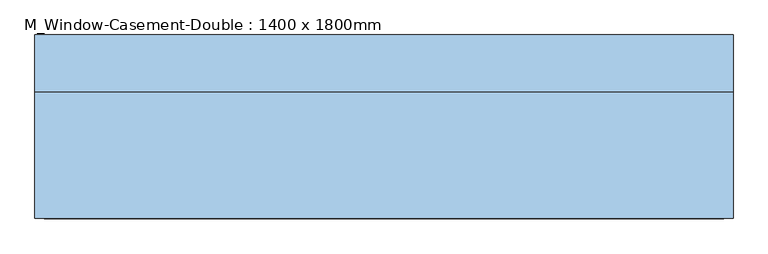
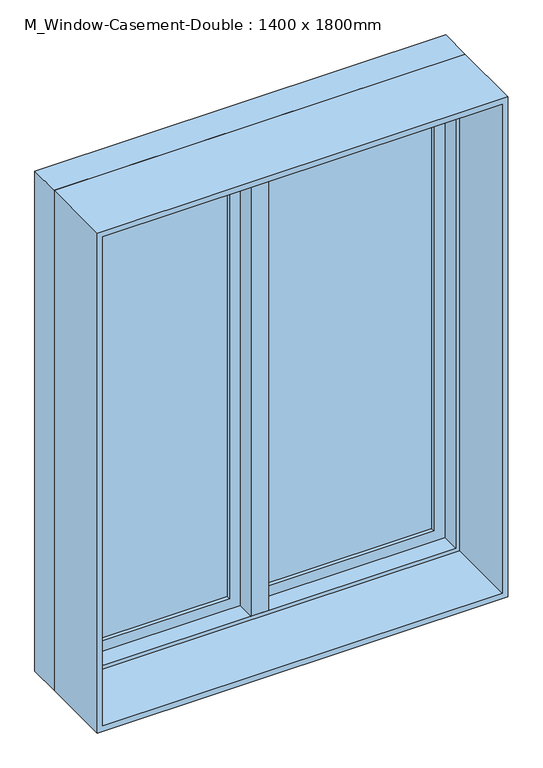
"""IFC4 building model written with IfcOpenShell, lengths in millimetres: window geometry, M_Window-Casement-Double : 1400 x 1800mm."""

from ifc_helpers import new_model, si_unit, frame, origin, place, context, project, spatial, polyline, outline, extrude, faceted_brep, source, transform, mapped, element, save


def m_window_casement_double_1400_x_1800mm_1c3ec30c(model_context):
    return source(origin(), model_context, "Body", "SolidModel", [
        faceted_brep([(668.25, 142.75, 2668.25), (668.25, 79.25, 2668.25), (-668.25, 79.25, 2668.25), (-668.25, 142.75, 2668.25), (687.3, 193.55, 2687.3), (687.3, 142.75, 2687.3), (-687.3, 142.75, 2687.3), (-687.3, 193.55, 2687.3), (700.0, 79.25, 2700.0), (700.0, 193.55, 2700.0), (-700.0, 193.55, 2700.0), (-700.0, 79.25, 2700.0), (-668.25, 79.25, 931.75), (-668.25, 142.75, 931.75), (-687.3, 142.75, 912.7), (-687.3, 193.55, 912.7), (-700.0, 193.55, 900.0), (-700.0, 79.25, 900.0), (668.25, 79.25, 931.75), (668.25, 142.75, 931.75), (687.3, 142.75, 912.7), (687.3, 193.55, 912.7), (700.0, 193.55, 900.0), (700.0, 79.25, 900.0)], [[[0, 1, 2, 3]], [[4, 5, 6, 7]], [[8, 9, 10, 11]], [[3, 2, 12, 13]], [[7, 6, 14, 15]], [[11, 10, 16, 17]], [[13, 12, 18, 19]], [[15, 14, 20, 21]], [[17, 16, 22, 23]], [[11, 17, 23, 8], [1, 18, 12, 2]], [[19, 18, 1, 0]], [[5, 20, 14, 6], [3, 13, 19, 0]], [[21, 20, 5, 4]], [[23, 22, 9, 8]], [[9, 22, 16, 10], [7, 15, 21, 4]]]),
        extrude(outline(polyline([(2700.0, -700.0), (900.0, -700.0), (900.0, 700.0), (2700.0, 700.0), (2700.0, -700.0)]), holes=[polyline([(2680.95, 680.95), (919.05, 680.95), (919.05, -680.95), (2680.95, -680.95), (2680.95, 680.95)])]), frame((0.0, -174.5, 0.0), z_axis=(0.0, 1.0, 0.0), x_axis=(0.0, 0.0, 1.0)), (0.0, 0.0, 1.0), 253.75),
        extrude(outline(polyline([(912.7, 687.3), (2687.3, 687.3), (2687.3, 9.525), (912.7, 9.525), (912.7, 687.3)]), holes=[polyline([(969.85, 66.675), (2630.15, 66.675), (2630.15, 630.15), (969.85, 630.15), (969.85, 66.675)])]), frame((0.0, 142.75, 0.0), z_axis=(0.0, 1.0, 0.0), x_axis=(0.0, 0.0, 1.0)), (0.0, 0.0, 1.0), 44.45),
        extrude(outline(polyline([(2687.3, -687.3), (912.7, -687.3), (912.7, -9.525), (2687.3, -9.525), (2687.3, -687.3)]), holes=[polyline([(2630.15, -66.675), (969.85, -66.675), (969.85, -630.15), (2630.15, -630.15), (2630.15, -66.675)])]), frame((0.0, 142.75, 0.0), z_axis=(0.0, 1.0, 0.0), x_axis=(0.0, 0.0, 1.0)), (0.0, 0.0, 1.0), 44.45),
        extrude(outline(polyline([(630.15, 174.5), (630.15, 168.15), (66.675, 168.15), (66.675, 174.5), (630.15, 174.5)])), frame((0.0, 0.0, 969.85), z_axis=(0.0, 0.0, 1.0), x_axis=(1.0, 0.0, 0.0)), (0.0, 0.0, 1.0), 1660.3),
        extrude(outline(polyline([(66.675, 155.45), (66.675, 161.8), (630.15, 161.8), (630.15, 155.45), (66.675, 155.45)])), frame((0.0, 0.0, 969.85), z_axis=(0.0, 0.0, 1.0), x_axis=(1.0, 0.0, 0.0)), (0.0, 0.0, 1.0), 1660.3),
        extrude(outline(polyline([(-66.675, 174.5), (-66.675, 168.15), (-630.15, 168.15), (-630.15, 174.5), (-66.675, 174.5)])), frame((0.0, 0.0, 969.85), z_axis=(0.0, 0.0, 1.0), x_axis=(1.0, 0.0, 0.0)), (0.0, 0.0, 1.0), 1660.3),
        extrude(outline(polyline([(-630.15, 155.45), (-630.15, 161.8), (-66.675, 161.8), (-66.675, 155.45), (-630.15, 155.45)])), frame((0.0, 0.0, 969.85), z_axis=(0.0, 0.0, 1.0), x_axis=(1.0, 0.0, 0.0)), (0.0, 0.0, 1.0), 1660.3),
        faceted_brep([(9.525, 193.55, 2687.3), (-9.525, 193.55, 2687.3), (-9.525, 142.75, 2687.3), (9.525, 142.75, 2687.3), (9.525, 193.55, 912.7), (9.525, 142.75, 912.7), (-9.525, 142.75, 912.7), (-9.525, 193.55, 912.7), (-9.525, 142.75, 931.75), (-9.525, 142.75, 2668.25), (-30.1625, 142.75, 931.75), (-30.1625, 142.75, 2668.25), (-30.1625, 79.25, 931.75), (-30.1625, 79.25, 2668.25), (30.1625, 79.25, 931.75), (30.1625, 79.25, 2668.25), (30.1625, 142.75, 931.75), (30.1625, 142.75, 2668.25), (9.525, 142.75, 931.75), (9.525, 142.75, 2668.25)], [[[0, 1, 2, 3]], [[4, 5, 6, 7]], [[1, 0, 4, 7]], [[2, 1, 7, 6, 8, 9]], [[9, 8, 10, 11]], [[11, 10, 12, 13]], [[13, 12, 14, 15]], [[15, 14, 16, 17]], [[17, 16, 18, 19]], [[0, 3, 19, 18, 5, 4]], [[18, 8, 6, 5]], [[9, 19, 3, 2]], [[8, 18, 16, 14, 12, 10]], [[19, 9, 11, 13, 15, 17]]]),
    ])


if __name__ == "__main__":
    model = new_model("IFC4")
    model_context = context("Model", 3, world=origin())
    ifc_project = project(units=[si_unit("LENGTHUNIT", "METRE", prefix="MILLI")], contexts=[model_context])
    site = spatial("IfcSite", under=ifc_project)
    building = spatial("IfcBuilding", under=site)
    placement = place(None, origin())
    m_window_casement_double_1400_x_1800mm_shape = m_window_casement_double_1400_x_1800mm_1c3ec30c(model_context)
    element("IfcWindow", 1, ObjectType="M_Window-Casement-Double : 1400 x 1800mm", at=placement, inside=building, context=model_context, shape_type="MappedRepresentation", body=[
        mapped(m_window_casement_double_1400_x_1800mm_shape, transform((0.0, 0.0, 0.0), x_axis=(1.0, 0.0, 0.0), y_axis=(0.0, 1.0, 0.0), z_axis=(0.0, 0.0, 1.0))),
    ])
    save(model, "model.ifc")

# Revit data of these elements
# Type "M_Window-Casement-Double : 1400 x 1800mm"
#   Type Mark = "27"
#   Fire Rating = "0.5h"
#   Assembly Code = "B2020100"
#   Analytic Construction = "Double glazing - domestic"
#   Frame Extension [instance default] = 6.35 mm
#   Window Inset [instance default] = 0 mm
#   Wall Thickness [instance default] = 150 mm
#   Interior Wall Closure [instance default] = 54.75 mm
#   Half Width = 700 mm
#   Visual Light Transmittance = 0.81
#   Thermal Resistance (R) = 0.319569 (m²·K)/W
#   Solar Heat Gain Coefficient = 0.76
#   Rough Width = 1415 mm
#   Rough Height = 1815 mm
#   Height = 1800 mm
#   Heat Transfer Coefficient (U) = 3.12929 W/(m²·K)
#   Exterior Wall Closure [instance default] = 31.8 mm
#   Extension Jamb [instance default] = 54.75 mm
#   Default Sill Height = 900 mm
#   Width = 1400 mm
#   Muntin Visibility = yes
#   Interior Trim Visibility [instance default] = yes
#   Exterior Trim Visibility [instance default] = yes
#   Extension Jamb Visibility [instance default] = yes
#   Interior Trim Material = Wood - Stained
#   Muntin Pattern = M_Muntin Pattern_2x2 : M_Muntin Pattern_2x2
#   Interior Trim = M_Trim-Window-Interior-Flat : Picture Frame
#   Interior Frame Material = Wood - Stained
#   Glass Panel Material = Glass
#   Exterior Trim Material = Clad - White
#   Exterior Trim = M_Trim-Window-Exterior-Flat : with Sill
#   Exterior Frame Material = Clad - White
#   Wall Closure = (empty or 0)
# Element 1 (IfcWindow, "M_Window-Casement-Double : 1400 x 1800mm")
#   Wall Thickness = 349 mm
#   Extension Jamb = 253.75 mm
#   Materials on its faces: "Wood - Stained", "Glass", "Clad - White"
# Materials
#   "Wood - Stained": class "Wood", colour RGB 173 132 96, transparency 0, Cost = 0
#   "Glass": class "Glass", colour RGB 245 245 243, transparency 1, Description = "Soda Lime Glass", Cost = 0
#   "Clad - White": class "Wood", colour RGB 245 245 243, transparency 0, Cost = 0
